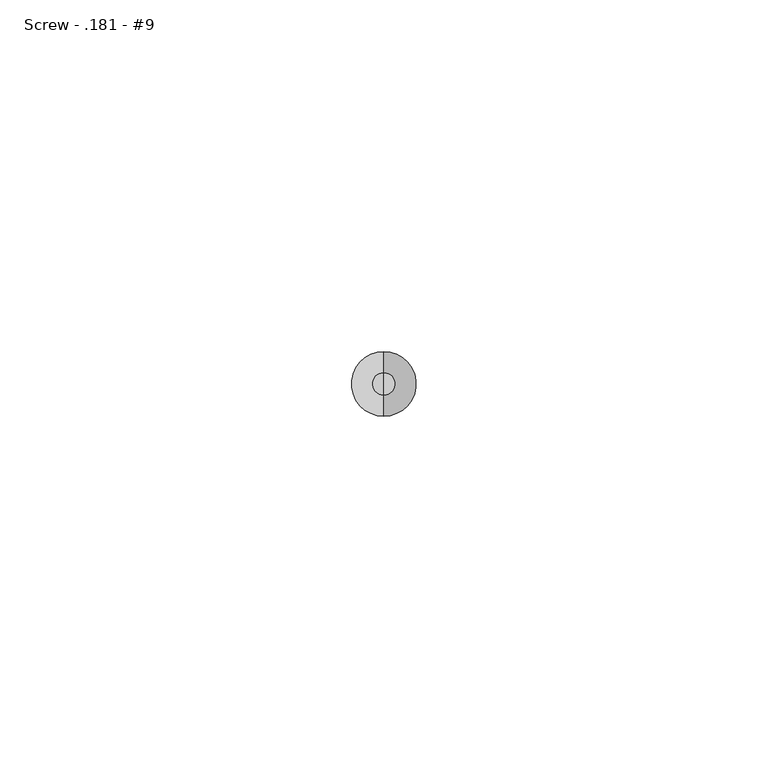
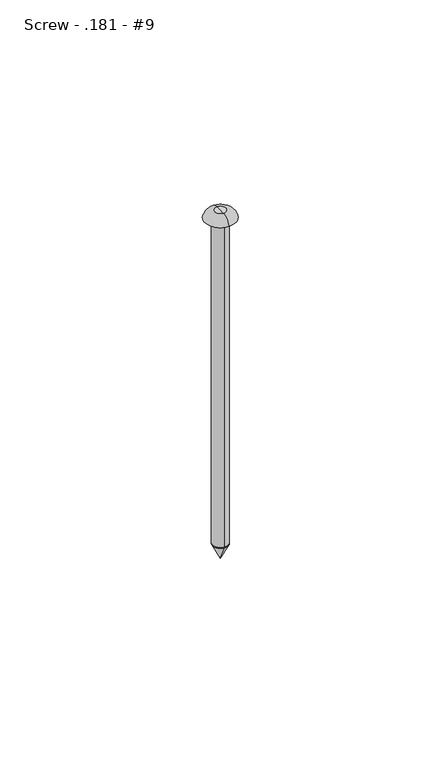
"""IFC4 building model written with IfcOpenShell, lengths in millimetres: fastener geometry, 060523 - W_P_C - Fastenings - Generic : Screw - .181 - #9."""

from ifc_helpers import new_model, si_unit, point, frame, origin, origin_2d, place, context, project, spatial, polyline, circle_curve, ellipse_curve, trimmed, segment, composite_curve, outline, extrude, source, transform, mapped, element, save
from ifc_brep_helpers import plane_surface, revolved_surface, advanced_brep


def screw_181_9_330bfe3c(model_context):
    return source(origin(), model_context, "Body", "SolidModel", [
        advanced_brep(
        [(0.0, -2.2987, -101.6), (0.0, 2.2987, -101.6), (0.0, 0.0, -101.6), (0.0, 0.0, -106.1974)],
        [
            (0, 1, circle_curve(frame((0.0, 0.0, -101.6), z_axis=(0.0, 0.0, 1.0), x_axis=(0.0, 1.0, 0.0)), 2.2987)),
            (1, 2),
            (2, 0),
            (1, 0, circle_curve(frame((0.0, 0.0, -101.6), z_axis=(0.0, 0.0, 1.0), x_axis=(0.0, 1.0, 0.0)), 2.2987)),
            (3, 1),
            (0, 3),
        ],
        [
            plane_surface(frame((0.0, 0.0, -101.6), z_axis=(0.0, 0.0, 1.0), x_axis=(0.0, 1.0, 0.0))),
            revolved_surface(polyline([(0.0, 2.2987, -101.6), (0.0, 0.0, -106.1974)]), (0.0, 0.0, -103.0840259), (0.0, 0.0, -1.0)),
        ],
        [
            (0, [[1, 2, 3]]),
            (0, [[4, -3, -2]]),
            (1, [[5, -1, 6]]),
            (1, [[-6, -4, -5]]),
        ],
    ),
        advanced_brep(
        [(0.0, 4.5974, 0.0), (0.0, -4.5974, 0.0), (0.0, 0.0, 0.0), (0.0, 0.0, 2.2987), (0.0, -1.5875, 2.2987), (0.0, 1.5875, 2.2987)],
        [
            (0, 1, circle_curve(frame((0.0, 0.0, 0.0), z_axis=(0.0, 0.0, -1.0), x_axis=(0.0, -1.0, 0.0)), 4.5974)),
            (1, 2),
            (2, 0),
            (1, 0, circle_curve(frame((0.0, 0.0, 0.0), z_axis=(0.0, 0.0, -1.0), x_axis=(0.0, -1.0, 0.0)), 4.5974)),
            (3, 4),
            (4, 5, circle_curve(frame((0.0, 0.0, 2.2987), z_axis=(0.0, 0.0, 1.0), x_axis=(0.0, -1.0, 0.0)), 1.5875)),
            (5, 3),
            (5, 4, circle_curve(frame((0.0, 0.0, 2.2987), z_axis=(0.0, 0.0, 1.0), x_axis=(0.0, -1.0, 0.0)), 1.5875)),
            (4, 1, circle_curve(frame((0.0, -1.5875, -0.8212199), z_axis=(1.0, 0.0, 0.0), x_axis=(0.0, -1.0, 0.0)), 3.1199199)),
            (0, 5, circle_curve(frame((0.0, 1.5875, -0.8212199), z_axis=(1.0, 0.0, 0.0), x_axis=(0.0, 1.0, 0.0)), 3.1199199)),
        ],
        [
            plane_surface(frame((0.0, 0.0, 0.0), z_axis=(0.0, 0.0, -1.0), x_axis=(0.0, -1.0, 0.0))),
            plane_surface(frame((0.0, 0.0, 2.2987), z_axis=(0.0, 0.0, 1.0), x_axis=(0.0, -1.0, 0.0))),
            revolved_surface(trimmed(ellipse_curve(frame((0.0, -1.5875, -0.8212199), z_axis=(-1.0, 0.0, 0.0), x_axis=(0.0, -1.0, 0.0)), 3.1199199, 3.1199199), [point((0.0, -4.5974, 0.0))], [point((0.0, -1.5875, 2.2987))], True, "CARTESIAN"), (0.0, 0.0, 1.4840259), (0.0, 0.0, 1.0)),
        ],
        [
            (0, [[1, 2, 3]]),
            (0, [[4, -3, -2]]),
            (1, [[5, 6, 7]]),
            (1, [[-7, 8, -5]]),
            (2, [[-6, 9, -1, 10]]),
            (2, [[-8, -10, -4, -9]]),
        ],
    ),
        extrude(outline(composite_curve([segment(trimmed(circle_curve(origin_2d(), 2.2987), [point((0.0, -2.2987))], [point((0.0, 2.2987))], False, "CARTESIAN"), True, "CONTINUOUS"), segment(trimmed(circle_curve(origin_2d(), 2.2987), [point((0.0, 2.2987))], [point((0.0, -2.2987))], False, "CARTESIAN"), True, "CONTINUOUS")], self_intersect=False)), frame((0.0, 0.0, -101.6), z_axis=(0.0, 0.0, 1.0), x_axis=(1.0, 0.0, 0.0)), (0.0, 0.0, 1.0), 101.6),
    ])


if __name__ == "__main__":
    model = new_model("IFC4")
    model_context = context("Model", 3, world=origin())
    ifc_project = project(units=[si_unit("LENGTHUNIT", "METRE", prefix="MILLI")], contexts=[model_context])
    site = spatial("IfcSite", under=ifc_project)
    building = spatial("IfcBuilding", under=site)
    placement = place(None, origin())
    screw_181_9_shape = screw_181_9_330bfe3c(model_context)
    element("IfcFastener", 1, ObjectType="060523 - W_P_C - Fastenings - Generic : Screw - .181 - #9", at=placement, inside=building, context=model_context, shape_type="MappedRepresentation", body=[
        mapped(screw_181_9_shape, transform((0.0, 0.0, 0.0), x_axis=(1.0, 0.0, 0.0), y_axis=(0.0, 1.0, 0.0), z_axis=(0.0, 0.0, 1.0))),
    ])
    save(model, "model.ifc")

# Revit data of these elements
# Type "060523 - W_P_C - Fastenings - Generic : Screw - .181 - #9"
#   Washer_Thickness = 0' - 0.00333"
#   Washer Radius = 0' - 0.1005"
#   Washer Offset - Head = 0' - 0"
#   Washer Offset = 0' - 0"
#   Thickness_of_Substrate [instance default] = 0' - 1"
#   Side = 0' - 0 37/64"
#   Radius = 0' - 0.0905"
#   Length [instance default] = 0' - 4"
#   Head Size = 0' - 1"
#   Head Radius = 0' - 0 1/2"
#   Head Height = 0' - 0.01"
#   Double Diameter = 0' - 0.362"
#   Diameter = 0' - 0.181"
#   Default Elevation = 4' - 0"
#   Washer_Nut_Visibility = no
#   Washer_Head_Visibility = no
#   Round_Head_Visibility = yes
#   Point Visibility = yes
#   Nut_Visibility = no
#   Hex_Head_Visiblilty = no
#   Washer Material = none
#   Bolt Material (Size) = AT SILL - FASTENER AT 24" O.C.
# Element 1 (IfcFastener, "060523 - W_P_C - Fastenings - Generic : Screw - .181 - #9")
#   Materials on its faces: "AT SILL - FASTENER AT 24\" O.C."
# Materials
#   "AT SILL - FASTENER AT 24\" O.C.": class "Generic", colour RGB 120 120 120, transparency 0, Cost = 0
